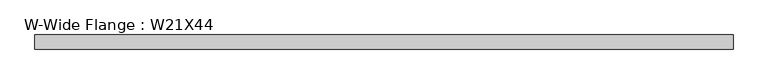
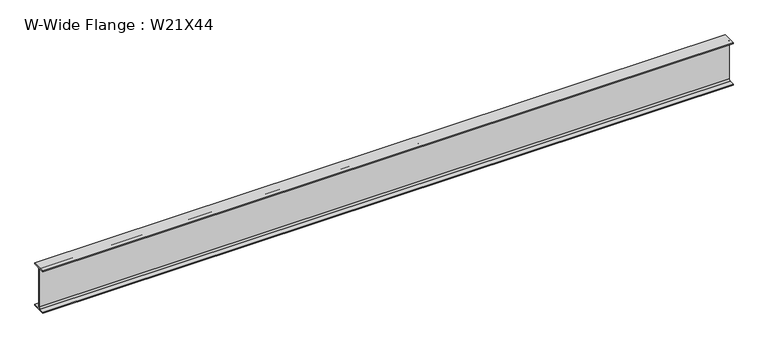
"""IFC4 building model written with IfcOpenShell, lengths in millimetres: beam geometry, W-Wide Flange : W21X44."""

from ifc_helpers import new_model, si_unit, point, frame, frame_2d, origin, place, context, project, spatial, polyline, circle_curve, trimmed, segment, composite_curve, outline, extrude, source, transform, mapped, element, save


def w_wide_flange_w21x44_9ef3883b(model_context):
    return source(origin(), model_context, "Body", "SweptSolid", [
        extrude(outline(composite_curve([segment(polyline([(82.55, -251.46), (82.55, -262.89), (-82.55, -262.89), (-82.55, -251.46), (-21.59, -251.46)]), True, "CONTINUOUS"), segment(trimmed(circle_curve(frame_2d((-21.59, -234.315)), 17.145), [point((-21.59, -251.46))], [point((-4.445, -234.315))], True, "CARTESIAN"), True, "CONTINUOUS"), segment(polyline([(-4.445, -234.315), (-4.445, 234.315)]), True, "CONTINUOUS"), segment(trimmed(circle_curve(frame_2d((-21.59, 234.315)), 17.145), [point((-4.445, 234.315))], [point((-21.59, 251.46))], True, "CARTESIAN"), True, "CONTINUOUS"), segment(polyline([(-21.59, 251.46), (-82.55, 251.46), (-82.55, 262.89), (82.55, 262.89), (82.55, 251.46), (21.59, 251.46)]), True, "CONTINUOUS"), segment(trimmed(circle_curve(frame_2d((21.59, 234.315)), 17.145), [point((21.59, 251.46))], [point((4.445, 234.315))], True, "CARTESIAN"), True, "CONTINUOUS"), segment(polyline([(4.445, 234.315), (4.445, -234.315)]), True, "CONTINUOUS"), segment(trimmed(circle_curve(frame_2d((21.59, -234.315)), 17.145), [point((4.445, -234.315))], [point((21.59, -251.46))], True, "CARTESIAN"), True, "CONTINUOUS"), segment(polyline([(21.59, -251.46), (82.55, -251.46)]), True, "CONTINUOUS")], self_intersect=False)), frame((-4076.7, 0.0, 0.0), z_axis=(1.0, 0.0, 0.0), x_axis=(0.0, 1.0, 0.0)), (0.0, 0.0, 1.0), 8153.4),
    ])


if __name__ == "__main__":
    model = new_model("IFC4")
    model_context = context("Model", 3, world=origin())
    ifc_project = project(units=[si_unit("LENGTHUNIT", "METRE", prefix="MILLI")], contexts=[model_context])
    site = spatial("IfcSite", under=ifc_project)
    building = spatial("IfcBuilding", under=site)
    placement = place(None, origin())
    w_wide_flange_w21x44_shape = w_wide_flange_w21x44_9ef3883b(model_context)
    element("IfcBeam", 1, ObjectType="W-Wide Flange : W21X44", at=placement, inside=building, context=model_context, shape_type="MappedRepresentation", body=[
        mapped(w_wide_flange_w21x44_shape, transform((0.0, 0.0, 0.0), x_axis=(1.0, 0.0, 0.0), y_axis=(0.0, 1.0, 0.0), z_axis=(0.0, 0.0, 1.0))),
    ])
    save(model, "model.ifc")

# Revit data of these elements
# Type "W-Wide Flange : W21X44"
#   Assembly Code = "B10"
#   W = 44
#   Length [instance default] = 5' - 0"
#   bf = 0' - 6 1/2"
#   d = 1' - 8.7"
#   k = 0' - 1 1/8"
#   k2 = 0' - 0.675"
#   tf = 0' - 0.45"
#   tw = 0' - 0.35"
#   A = 0.0902778 SF
#   Structural Material [instance default] = Steel ASTM A992
# Element 1 (IfcBeam, "W-Wide Flange : W21X44")
#   Materials on its faces: "Steel ASTM A992"
# Materials
#   "Steel ASTM A992": class "Metal", colour RGB 199 199 199, transparency 0, Description = "Structural steel 50ksi", Cost = 0
